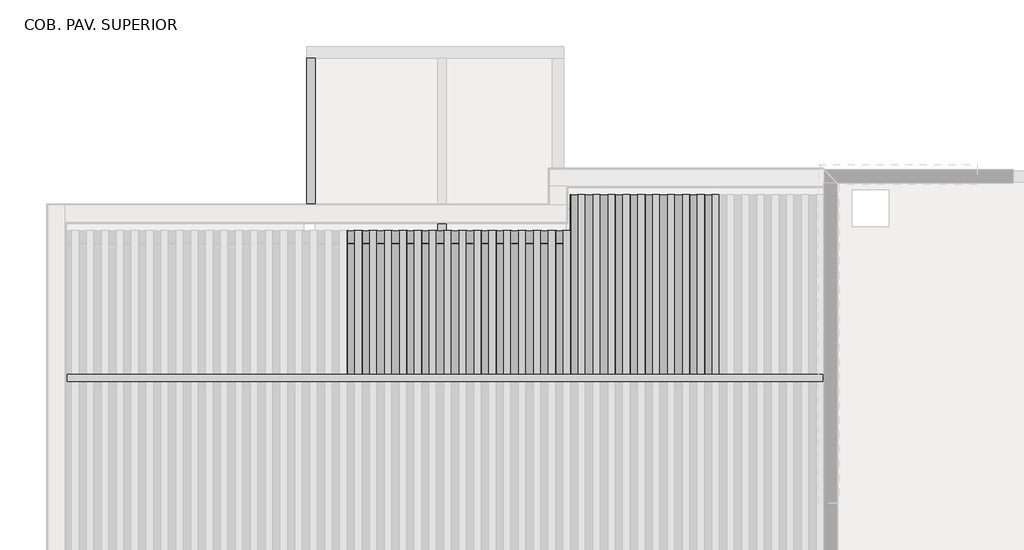
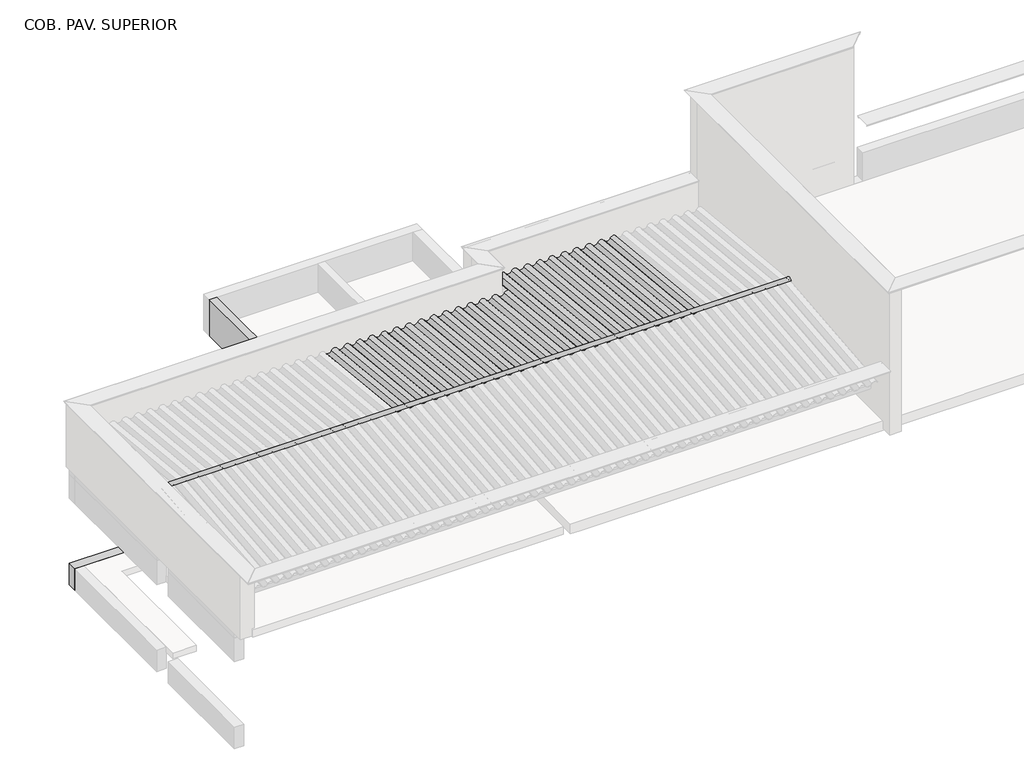
# One storey, part 4 of 7: 41 beams, 9 columns.
"""IFC4 building model written with IfcOpenShell, lengths in millimetres."""

import ifcopenshell
import ifcopenshell.guid

model = None  # the IFC model being written
_history = None  # IfcOwnerHistory: only IFC2X3 demands one
_inside = {}  # id of a spatial element -> (the spatial element, [elements in it])
_under = {}  # id of a project, library or spatial element -> (it, [spatial elements below it])
_declared = {}  # id of a project -> (the project, [libraries it declares])
_typed = {}  # id of a type object -> (the type object, [elements of that type])
_made_of = {}  # id of a material, layer set ... -> (it, [elements and type objects made of it])


def new_model(schema):
    """Start an empty IFC model of exactly this schema.

    Asked for "IFC4X3", IfcOpenShell would pick the latest addendum, in which some entities
    have other attributes; the version numbers below select the first issue.
    IFC2X3 requires an IfcOwnerHistory on every rooted entity: one is made here for all.
    """
    global model, _history
    if schema == "IFC4X3":
        model = ifcopenshell.file(schema_version=(4, 3, 0, 0))
    else:
        model = ifcopenshell.file(schema=schema)
    _inside.clear()
    _under.clear()
    _declared.clear()
    _typed.clear()
    _made_of.clear()
    _history = None
    if model.schema == "IFC2X3":
        org = make("IfcOrganization", Name="unknown")
        user = make(
            "IfcPersonAndOrganization",
            ThePerson=make("IfcPerson", FamilyName="unknown"),
            TheOrganization=org,
        )
        app = make(
            "IfcApplication",
            ApplicationDeveloper=org,
            Version="unknown",
            ApplicationFullName="unknown",
            ApplicationIdentifier="unknown",
        )
        _history = make(
            "IfcOwnerHistory",
            OwningUser=user,
            OwningApplication=app,
            ChangeAction="ADDED",
            CreationDate=0,
        )
    return model


def make(cls, **values):
    """One entity of the class cls with the attributes given. An attribute that is None is left unset."""
    return model.create_entity(
        cls, **{name: value for name, value in values.items() if value is not None}
    )


def rooted(cls, **values):
    """An entity with a GlobalId (a new one), such as an element, a storey or a relation."""
    return make(cls, GlobalId=ifcopenshell.guid.new(), OwnerHistory=_history, **values)


def si_unit(unit_type, name, prefix=None):
    """IfcSIUnit, for example si_unit("LENGTHUNIT", "METRE", prefix="MILLI")."""
    return make("IfcSIUnit", UnitType=unit_type, Prefix=prefix, Name=name)


def assignment(units):
    """IfcUnitAssignment: the units of a project."""
    return None if units is None else make("IfcUnitAssignment", Units=units)


def point(xyz):
    """IfcCartesianPoint."""
    return None if xyz is None else make("IfcCartesianPoint", Coordinates=xyz)


def direction(xyz):
    """IfcDirection."""
    return None if xyz is None else make("IfcDirection", DirectionRatios=xyz)


def frame(location, z_axis=None, x_axis=None):
    """IfcAxis2Placement3D, a coordinate frame: its origin and axes. An axis left out is left unset."""
    return make(
        "IfcAxis2Placement3D",
        Location=point(location),
        Axis=direction(z_axis),
        RefDirection=direction(x_axis),
    )


def frame_2d(location, x_axis=None):
    """IfcAxis2Placement2D, a coordinate frame in the plane: its origin and x axis."""
    return make(
        "IfcAxis2Placement2D", Location=point(location), RefDirection=direction(x_axis)
    )


def origin():
    """The frame at (0, 0, 0) with its axes left unset."""
    return frame((0.0, 0.0, 0.0))


def place(relative_to, where):
    """IfcLocalPlacement: puts the frame where relative to a parent placement (None: the world)."""
    return make(
        "IfcLocalPlacement", PlacementRelTo=relative_to, RelativePlacement=where
    )


def context(
    kind, dimensions, precision=None, world=None, true_north=None, identifier=None
):
    """IfcGeometricRepresentationContext, for example the 3D "Model" context."""
    return make(
        "IfcGeometricRepresentationContext",
        ContextIdentifier=identifier,
        ContextType=kind,
        CoordinateSpaceDimension=dimensions,
        Precision=precision,
        WorldCoordinateSystem=world,
        TrueNorth=true_north,
    )


def project(units=None, contexts=None):
    """IfcProject with its units and contexts."""
    return rooted(
        "IfcProject",
        Name="project",
        RepresentationContexts=contexts,
        UnitsInContext=assignment(units),
    )


def spatial(cls, under=None, at=None, **own):
    """A site, building, storey or space (cls), placed at a placement, below another one or the project."""
    s = rooted(cls, ObjectPlacement=at, **own)
    if under is not None:
        _under.setdefault(under.id(), (under, []))[1].append(s)
    return s


def polyline(points):
    """IfcPolyline through the points."""
    return make("IfcPolyline", Points=[point(p) for p in points])


def circle_curve(where, radius):
    """IfcCircle in the frame where."""
    return make("IfcCircle", Position=where, Radius=radius)


def trimmed(basis, trim1, trim2, sense, master):
    """IfcTrimmedCurve: the piece of a basis curve between two trims."""
    return make(
        "IfcTrimmedCurve",
        BasisCurve=basis,
        Trim1=trim1,
        Trim2=trim2,
        SenseAgreement=sense,
        MasterRepresentation=master,
    )


def segment(curve, same_sense, transition):
    """IfcCompositeCurveSegment."""
    return make(
        "IfcCompositeCurveSegment",
        Transition=transition,
        SameSense=same_sense,
        ParentCurve=curve,
    )


def composite_curve(segments, self_intersect=None):
    """IfcCompositeCurve: segments joined end to end."""
    return make("IfcCompositeCurve", Segments=segments, SelfIntersect=self_intersect)


def outline(outer, holes=None, kind="AREA"):
    """IfcArbitraryClosedProfileDef: a profile drawn as a closed curve; with holes, ...WithVoids."""
    if holes is None:
        return make("IfcArbitraryClosedProfileDef", ProfileType=kind, OuterCurve=outer)
    return make(
        "IfcArbitraryProfileDefWithVoids",
        ProfileType=kind,
        OuterCurve=outer,
        InnerCurves=holes,
    )


def extrude(swept, where, along, depth):
    """IfcExtrudedAreaSolid: the profile swept, set in the frame where, extruded along a direction by depth."""
    return make(
        "IfcExtrudedAreaSolid",
        SweptArea=swept,
        Position=where,
        ExtrudedDirection=direction(along),
        Depth=depth,
    )


def faces_of(points, faces, orient=None, outer=None):
    """IfcFace entities. A face is a list of loops; a loop is a list of indices into points, from 0.

    orient and outer hold one flag for each loop. By default every Orientation is true, the
    first loop of a face is its IfcFaceOuterBound and the others are IfcFaceBound.
    """
    made = []
    for i, loops in enumerate(faces):
        bounds = []
        for j, loop in enumerate(loops):
            is_outer = j == 0 if outer is None else outer[i][j]
            bounds.append(
                make(
                    "IfcFaceOuterBound" if is_outer else "IfcFaceBound",
                    Bound=make("IfcPolyLoop", Polygon=[points[k] for k in loop]),
                    Orientation=True if orient is None else orient[i][j],
                )
            )
        made.append(make("IfcFace", Bounds=bounds))
    return made


def faceted_brep(points, faces, orient=None, outer=None, voids=None):
    """IfcFacetedBrep: a solid bounded by flat faces; with voids (closed shells), ...WithVoids."""
    shared = [point(p) for p in points]
    hull = make("IfcClosedShell", CfsFaces=faces_of(shared, faces, orient, outer))
    if voids is None:
        return make("IfcFacetedBrep", Outer=hull)
    return make(
        "IfcFacetedBrepWithVoids",
        Outer=hull,
        Voids=[
            make(cls, CfsFaces=faces_of(shared, fs, o, b)) for cls, fs, o, b in voids
        ],
    )


def shape(context_of_items, identifier, shape_type, items):
    """IfcShapeRepresentation: the items that make up one representation, for example the "Body"."""
    return make(
        "IfcShapeRepresentation",
        ContextOfItems=context_of_items,
        RepresentationIdentifier=identifier,
        RepresentationType=shape_type,
        Items=items,
    )


def source(mapping_origin, context_of_items, identifier, shape_type, items):
    """IfcRepresentationMap: a shape defined once, which mapped items show again and again."""
    return make(
        "IfcRepresentationMap",
        MappingOrigin=mapping_origin,
        MappedRepresentation=shape(context_of_items, identifier, shape_type, items),
    )


def transform(
    local_origin,
    x_axis=None,
    y_axis=None,
    z_axis=None,
    scale=None,
    scale2=None,
    scale3=None,
    uniform=True,
):
    """IfcCartesianTransformationOperator3D, or its non-uniform kind. x_axis, y_axis, z_axis: its Axis1, 2, 3."""
    if uniform:
        return make(
            "IfcCartesianTransformationOperator3D",
            Axis1=direction(x_axis),
            Axis2=direction(y_axis),
            LocalOrigin=point(local_origin),
            Scale=scale,
            Axis3=direction(z_axis),
        )
    return make(
        "IfcCartesianTransformationOperator3DnonUniform",
        Axis1=direction(x_axis),
        Axis2=direction(y_axis),
        LocalOrigin=point(local_origin),
        Scale=scale,
        Axis3=direction(z_axis),
        Scale2=scale2,
        Scale3=scale3,
    )


def mapped(mapping_source, mapping_target):
    """IfcMappedItem: shows the shape of a source again, moved by a transform."""
    return make(
        "IfcMappedItem", MappingSource=mapping_source, MappingTarget=mapping_target
    )


def made_of(thing, what):
    """Note that an element or type object is made of a material, layer set ...; save() writes the relation."""
    if what is not None:
        _made_of.setdefault(what.id(), (what, []))[1].append(thing)
    return thing


def element(
    cls,
    number,
    at=None,
    inside=None,
    cuts=None,
    type_object=None,
    material=None,
    context=None,
    identifier="Body",
    shape_type=None,
    held_by="IfcProductDefinitionShape",
    body=None,
    shapes=None,
    **own,
):
    """One element of the class cls, such as IfcWall. Its Tag is "e" and its number.

    at: its placement. inside: the storey or other place that contains it. cuts: it is an
    opening in that element (IfcRelVoidsElement). A single representation is given by context,
    identifier, shape_type and body (its items); several are given by shapes. held_by: the class
    of the entity that holds the representations. save() writes the other relations.
    """
    e = rooted(cls, Tag="e%d" % number, ObjectPlacement=at, **own)
    if body is not None:
        shapes = [shape(context, identifier, shape_type, body)]
    if shapes is not None:
        e.Representation = make(held_by, Representations=shapes)
    if inside is not None:
        _inside.setdefault(inside.id(), (inside, []))[1].append(e)
    if cuts is not None:
        rooted(
            "IfcRelVoidsElement", RelatingBuildingElement=cuts, RelatedOpeningElement=e
        )
    if type_object is not None:
        _typed.setdefault(type_object.id(), (type_object, []))[1].append(e)
    return made_of(e, material)


def aggregate(whole, parts):
    """IfcRelAggregates: a whole, such as a stair, and the parts it consists of."""
    return rooted("IfcRelAggregates", RelatingObject=whole, RelatedObjects=parts)


def save(model, path):
    """Write the relations noted so far, then the file.

    IfcRelAggregates (storeys below a building ...), IfcRelContainedInSpatialStructure (elements
    in a storey), IfcRelDefinesByType, IfcRelAssociatesMaterial and IfcRelDeclares: one each for
    every whole, place, type object, material and project.
    """
    for whole, parts in _under.values():
        aggregate(whole, parts)
    for where, things in _inside.values():
        rooted(
            "IfcRelContainedInSpatialStructure",
            RelatedElements=things,
            RelatingStructure=where,
        )
    for kind, things in _typed.values():
        rooted("IfcRelDefinesByType", RelatedObjects=things, RelatingType=kind)
    for what, things in _made_of.values():
        rooted("IfcRelAssociatesMaterial", RelatedObjects=things, RelatingMaterial=what)
    for by, libraries in _declared.values():
        rooted("IfcRelDeclares", RelatingContext=by, RelatedDefinitions=libraries)
    model.write(path)


def cumeeira_telha_ondulada_fibrocimento_4a9e66c1(model_context):
    return source(origin(), model_context, "Body", "SweptSolid", [
        extrude(outline(composite_curve([segment(polyline([(58.3970135, 42.4437972), (53.9055884, 40.2467307)]), True, "CONTINUOUS"), segment(trimmed(circle_curve(frame_2d((-1.6029865, 13.0936483)), 61.7939461), [point((53.9055884, 40.2467307))], [point((-57.1115615, 40.2467307))], True, "CARTESIAN"), True, "CONTINUOUS"), segment(polyline([(-57.1115615, 40.2467307), (-61.6029865, 42.4437972)]), True, "CONTINUOUS"), segment(trimmed(circle_curve(frame_2d((-1.6029865, 13.0936483)), 66.7939461), [point((-61.6029865, 42.4437972))], [point((58.3970135, 42.4437972))], False, "CARTESIAN"), True, "CONTINUOUS")], self_intersect=False)), frame((-6200.0, 0.0, 0.0), z_axis=(1.0, 0.0, 0.0), x_axis=(0.0, 1.0, 0.0)), (0.0, 0.0, 1.0), 12400.0),
    ])


def viga_cumeeira_6x16cm_b61bb166(model_context):
    return source(origin(), model_context, "Body", "SweptSolid", [
        extrude(outline(polyline([(6210.0, 30.0), (6210.0, -30.0), (-6210.0, -30.0), (-6210.0, 30.0), (6210.0, 30.0)])), frame((0.0, 0.0, -80.0), z_axis=(0.0, 0.0, 1.0), x_axis=(1.0, 0.0, 0.0)), (0.0, 0.0, 1.0), 160.0),
    ])


def column_d505325c(model_context):
    return source(origin(), model_context, "Body", "SweptSolid", [
        extrude(outline(polyline([(30.0, 80.0), (30.0, -80.0), (-30.0, -80.0), (-30.0, 80.0), (30.0, 80.0)])), frame((0.0, 0.0, 6710.0), z_axis=(0.0, 0.0, 1.0), x_axis=(1.0, 0.0, 0.0)), (0.0, 0.0, 1.0), 750.0),
    ])


def column_df674f92(model_context):
    return source(origin(), model_context, "Body", "SweptSolid", [
        extrude(outline(polyline([(30.0, 80.0), (30.0, -80.0), (-30.0, -80.0), (-30.0, 80.0), (30.0, 80.0)])), frame((0.0, 0.0, 6710.0), z_axis=(0.0, 0.0, 1.0), x_axis=(1.0, 0.0, 0.0)), (0.0, 0.0, 1.0), 575.0),
    ])


def column_4db371bd(model_context):
    return source(origin(), model_context, "Body", "SweptSolid", [
        extrude(outline(polyline([(30.0, 80.0), (30.0, -80.0), (-30.0, -80.0), (-30.0, 80.0), (30.0, 80.0)])), frame((0.0, 0.0, 6710.0), z_axis=(0.0, 0.0, 1.0), x_axis=(1.0, 0.0, 0.0)), (0.0, 0.0, 1.0), 660.0),
    ])


model = new_model("IFC4")

# Units and contexts
model_context = context("Model", 3, world=origin())
ifc_project = project(units=[si_unit("LENGTHUNIT", "METRE", prefix="MILLI")], contexts=[model_context])

# Site, building, storey
site = spatial("IfcSite", under=ifc_project)
building = spatial("IfcBuilding", under=site)
storey = spatial("IfcBuildingStorey", under=building, Name="COB. PAV. SUPERIOR", Elevation=6650.0)

# Beams
placement = place(None, origin())
element("IfcBeam", 1, at=placement, inside=storey, context=model_context, shape_type="SweptSolid", body=[
    extrude(outline(polyline([(-6679.281307, -7711.5607799), (-6679.281307, -7831.5607799), (-8679.281307, -7831.5607799), (-8679.281307, -7711.5607799), (-6679.281307, -7711.5607799)])), frame((0.0, 0.0, 6650.0), z_axis=(0.0, 0.0, 1.0), x_axis=(1.0, 0.0, 0.0)), (0.0, 0.0, 1.0), 60.0),
])
element("IfcBeam", 2, at=placement, inside=storey, context=model_context, shape_type="SweptSolid", body=[
    extrude(outline(polyline([(-4679.281307, -7711.5607799), (-4679.281307, -7831.5607799), (-6679.281307, -7831.5607799), (-6679.281307, -7711.5607799), (-4679.281307, -7711.5607799)])), frame((0.0, 0.0, 6650.0), z_axis=(0.0, 0.0, 1.0), x_axis=(1.0, 0.0, 0.0)), (0.0, 0.0, 1.0), 60.0),
])
element("IfcBeam", 3, at=placement, inside=storey, context=model_context, shape_type="SweptSolid", body=[
    extrude(outline(polyline([(-2679.281307, -7711.5607799), (-2679.281307, -7831.5607799), (-4679.281307, -7831.5607799), (-4679.281307, -7711.5607799), (-2679.281307, -7711.5607799)])), frame((0.0, 0.0, 6650.0), z_axis=(0.0, 0.0, 1.0), x_axis=(1.0, 0.0, 0.0)), (0.0, 0.0, 1.0), 60.0),
])
element("IfcBeam", 4, at=placement, inside=storey, context=model_context, shape_type="SweptSolid", body=[
    extrude(outline(polyline([(-8779.281307, -5488.3211004), (-8779.281307, -5608.3211004), (-10679.281307, -5608.3211004), (-10679.281307, -5488.3211004), (-8779.281307, -5488.3211004)])), frame((0.0, 0.0, 6650.0), z_axis=(0.0, 0.0, 1.0), x_axis=(1.0, 0.0, 0.0)), (0.0, 0.0, 1.0), 60.0),
])
element("IfcBeam", 5, at=placement, inside=storey, context=model_context, shape_type="SweptSolid", body=[
    extrude(outline(polyline([(-6779.2813076, -5488.3211004), (-6779.2813076, -5608.3211004), (-8589.281307, -5608.3211004), (-8589.281307, -5488.3211004), (-6779.2813076, -5488.3211004)])), frame((0.0, 0.0, 6650.0), z_axis=(0.0, 0.0, 1.0), x_axis=(1.0, 0.0, 0.0)), (0.0, 0.0, 1.0), 60.0),
])
element("IfcBeam", 6, at=placement, inside=storey, context=model_context, shape_type="SweptSolid", body=[
    extrude(outline(polyline([(-4779.281307, -5488.3211004), (-4779.281307, -5608.3211004), (-6779.2813063, -5608.3211004), (-6779.2813063, -5488.3211004), (-4779.281307, -5488.3211004)])), frame((0.0, 0.0, 6650.0), z_axis=(0.0, 0.0, 1.0), x_axis=(1.0, 0.0, 0.0)), (0.0, 0.0, 1.0), 60.0),
])
element("IfcBeam", 7, at=placement, inside=storey, context=model_context, shape_type="SweptSolid", body=[
    extrude(outline(polyline([(-6840.281307, -6319.8711004), (-6840.281307, -6439.8711004), (-8589.281307, -6439.8711004), (-8589.281307, -6319.8711004), (-6840.281307, -6319.8711004)])), frame((0.0, 0.0, 6650.0), z_axis=(0.0, 0.0, 1.0), x_axis=(1.0, 0.0, 0.0)), (0.0, 0.0, 1.0), 60.0),
])
element("IfcBeam", 8, at=placement, inside=storey, context=model_context, shape_type="SweptSolid", body=[
    extrude(outline(polyline([(-4679.2813076, -6319.8711004), (-4679.2813076, -6439.8711004), (-6440.281307, -6439.8711004), (-6440.281307, -6319.8711004), (-4679.2813076, -6319.8711004)])), frame((0.0, 0.0, 6650.0), z_axis=(0.0, 0.0, 1.0), x_axis=(1.0, 0.0, 0.0)), (0.0, 0.0, 1.0), 60.0),
])
element("IfcBeam", 9, at=placement, inside=storey, context=model_context, shape_type="SweptSolid", body=[
    extrude(outline(polyline([(-2679.2813076, -6319.8711004), (-2679.2813076, -6439.8711004), (-4679.2813064, -6439.8711004), (-4679.2813064, -6319.8711004), (-2679.2813076, -6319.8711004)])), frame((0.0, 0.0, 6650.0), z_axis=(0.0, 0.0, 1.0), x_axis=(1.0, 0.0, 0.0)), (0.0, 0.0, 1.0), 60.0),
])
cumeeira_telha_ondulada_fibrocimento_shape = cumeeira_telha_ondulada_fibrocimento_4a9e66c1(model_context)
element("IfcBeam", 10, ObjectType="Cumeeira Telha Ondulada : Fibrocimento", at=placement, inside=storey, context=model_context, shape_type="MappedRepresentation", body=[
    mapped(cumeeira_telha_ondulada_fibrocimento_shape, transform((-6459.6793166, -7771.5607799, 7660.6251229), x_axis=(-1.0, 0.0, 0.0), y_axis=(0.0, -1.0, 0.0), z_axis=(0.0, 0.0, 1.0))),
])
element("IfcBeam", 11, ObjectType="TQS - Viga retangular : 14.0 x 76.0", at=placement, inside=storey, context=model_context, shape_type="Brep", body=[
    faceted_brep([(-8730.281307, -4975.5699847, 7050.0), (-8590.281307, -4975.5699847, 7050.0), (-8590.281307, -2515.5699847, 7050.0), (-8730.281307, -2515.5699847, 7050.0), (-8590.281307, -4975.5699847, 6450.0), (-8590.281307, -4975.5699847, 6290.0), (-8590.281307, -2515.5699847, 6290.0), (-8590.281307, -2515.5699847, 6450.0), (-8730.281307, -4975.5699847, 6290.0), (-8730.281307, -2515.5699847, 6290.0)], [[[0, 1, 2, 3]], [[1, 4, 5, 6, 7, 2]], [[5, 8, 9, 6]], [[8, 0, 3, 9]], [[1, 0, 8, 5, 4]], [[3, 2, 7, 6, 9]]]),
])
element("IfcBeam", 12, ObjectType="TQS - Viga retangular : 14.0 x 76.0", at=placement, inside=storey, context=model_context, shape_type="Brep", body=[
    faceted_brep([(-6440.281307, -5165.5699847, 7050.0), (-6580.281307, -5165.5699847, 7050.0), (-6580.281307, -6413.3699847, 7050.0), (-6440.281307, -6413.3699847, 7050.0), (-6440.281307, -5165.5699847, 6290.0), (-6440.281307, -5165.5699847, 6450.0), (-6440.281307, -5165.5699847, 6650.0), (-6440.281307, -6413.3699847, 6290.0), (-6580.281307, -5165.5699847, 6290.0), (-6580.281307, -6413.3699847, 6290.0), (-6580.281307, -5165.5699847, 6450.0), (-6580.281307, -6413.3699847, 6450.0)], [[[0, 1, 2, 3]], [[4, 5, 6, 0, 3, 7]], [[8, 4, 7, 9]], [[1, 10, 8, 9, 11, 2]], [[1, 0, 6, 5, 4, 8, 10]], [[2, 11, 9, 7, 3]]]),
])
element("IfcBeam", 13, ObjectType="TQS - Viga retangular : 19.0 x 45.0", at=placement, inside=storey, context=model_context, shape_type="Brep", body=[
    faceted_brep([(-8779.281307, -5165.5699847, 4480.0), (-8779.281307, -4975.5699847, 4480.0), (-12930.2813069, -4975.5699847, 4480.0), (-12930.2813069, -5165.5699847, 4480.0), (-12740.2813069, -5165.5699847, 4480.0), (-9711.481307, -5165.5699847, 4480.0), (-8779.281307, -5165.5699847, 4030.0), (-12930.2813069, -5165.5699847, 4030.0), (-12740.2813069, -5165.5699847, 4030.0), (-8779.281307, -4975.5699847, 4030.0), (-12930.2813069, -4975.5699847, 4030.0)], [[[0, 1, 2, 3, 4, 5]], [[6, 0, 5, 4, 3, 7, 8]], [[9, 6, 8, 7, 10]], [[1, 9, 10, 2]], [[1, 0, 6, 9]], [[3, 2, 10, 7]]]),
])
element("IfcBeam", 14, ObjectType="TQS - Viga retangular : 19.0 x 96.0", at=placement, inside=storey, context=model_context, shape_type="Brep", body=[
    faceted_brep([(-4702.281307, -5165.5699847, 7250.0), (-4512.281307, -5165.5699847, 7250.0), (-4512.281307, -4565.5699847, 7250.0), (-4512.281307, -4375.5699847, 7250.0), (-4702.281307, -4375.5699847, 7250.0), (-4702.281307, -4975.5699847, 7250.0), (-4512.281307, -4375.5699847, 6290.0), (-4512.281307, -4375.5699847, 6450.0), (-4512.281307, -4375.5699847, 7050.0), (-4512.281307, -5165.5699847, 6650.0), (-4512.281307, -5165.5699847, 6450.0), (-4512.281307, -5165.5699847, 6290.0), (-4702.281307, -5165.5699847, 6290.0), (-4702.281307, -4975.5699847, 6290.0), (-4702.281307, -4375.5699847, 6290.0), (-4702.281307, -4375.5699847, 7050.0), (-4702.281307, -5165.5699847, 6450.0), (-4702.281307, -5165.5699847, 6650.0)], [[[0, 1, 2, 3, 4, 5]], [[6, 7, 8, 3, 2, 1, 9, 10, 11]], [[11, 12, 13, 14, 6]], [[4, 15, 14, 13, 12, 16, 17, 0, 5]], [[1, 0, 17, 16, 12, 11, 10, 9]], [[4, 3, 8, 7, 6, 14, 15]]]),
])
element("IfcBeam", 15, ObjectType="TQS - Viga retangular : 19.0 x 96.0", at=placement, inside=storey, context=model_context, shape_type="Brep", body=[
    faceted_brep([(-6440.281307, -4975.5699847, 7250.0), (-6440.281307, -5165.5699847, 7250.0), (-4702.281307, -5165.5699847, 7250.0), (-4702.281307, -4975.5699847, 7250.0), (-6440.281307, -5165.5699847, 6650.0), (-6440.281307, -5165.5699847, 6450.0), (-6440.281307, -5165.5699847, 6290.0), (-4702.281307, -5165.5699847, 6290.0), (-4702.281307, -5165.5699847, 6450.0), (-4702.281307, -5165.5699847, 6650.0), (-6440.281307, -4975.5699847, 6290.0), (-4702.281307, -4975.5699847, 6290.0), (-6440.281307, -4975.5699847, 6450.0), (-4702.281307, -4975.5699847, 6450.0)], [[[0, 1, 2, 3]], [[2, 1, 4, 5, 6, 7, 8, 9]], [[6, 10, 11, 7]], [[10, 12, 0, 3, 13, 11]], [[1, 0, 12, 10, 6, 5, 4]], [[3, 2, 9, 8, 7, 11, 13]]]),
    faceted_brep([(-8589.281307, -5165.5699847, 7250.0), (-8589.281307, -4975.5699847, 7250.0), (-8589.281307, -4975.5699847, 6290.0), (-8589.281307, -5165.5699847, 6290.0), (-8589.281307, -5165.5699847, 6450.0), (-6630.281307, -4975.5699847, 7250.0), (-6630.281307, -5165.5699847, 7250.0), (-6630.281307, -5165.5699847, 6290.0), (-6630.281307, -4975.5699847, 6290.0)], [[[0, 1, 2, 3, 4]], [[5, 6, 7, 8]], [[1, 0, 6, 5]], [[0, 4, 3, 7, 6]], [[3, 2, 8, 7]], [[2, 1, 5, 8]]]),
])
element("IfcBeam", 16, ObjectType="Telha Ondulada : Fibrocimento", at=placement, inside=storey, context=model_context, shape_type="SweptSolid", body=[
    extrude(outline(composite_curve([segment(trimmed(circle_curve(frame_2d((-58.7002978, -53.2060539)), 66.7939461), [point((-29.3501489, 6.7939461))], [point((-29.3501489, -113.2060539))], False, "CARTESIAN"), True, "CONTINUOUS"), segment(polyline([(-29.3501489, -113.2060539), (-31.5472154, -108.7146289)]), True, "CONTINUOUS"), segment(trimmed(circle_curve(frame_2d((-58.7002978, -53.2060539)), 61.7939461), [point((-31.5472154, -108.7146289))], [point((-31.5472154, 2.3025211))], True, "CARTESIAN"), True, "CONTINUOUS"), segment(trimmed(circle_curve(frame_2d((0.0, 66.7939461)), 71.7939461), [point((-31.5472154, 2.3025211))], [point((-31.5472154, 131.2853711))], False, "CARTESIAN"), True, "CONTINUOUS"), segment(polyline([(-31.5472154, 131.2853711), (-29.3501489, 126.7939461)]), True, "CONTINUOUS"), segment(trimmed(circle_curve(frame_2d((0.0, 66.7939461)), 66.7939461), [point((-29.3501489, 126.7939461))], [point((-29.3501489, 6.7939461))], True, "CARTESIAN"), True, "CONTINUOUS")], self_intersect=False)), frame((-7939.8843743, -5348.1805671, 7453.4315886), z_axis=(0.0, -0.9950371902099893, 0.09950371902099772), x_axis=(0.0, 0.09950371902099772, 0.9950371902099893)), (0.0, 0.0, 1.0), 2425.2918406),
])
element("IfcBeam", 17, ObjectType="Telha Ondulada : Fibrocimento", at=placement, inside=storey, context=model_context, shape_type="SweptSolid", body=[
    extrude(outline(composite_curve([segment(trimmed(circle_curve(frame_2d((-58.7002978, -53.2060539)), 66.7939461), [point((-29.3501489, 6.7939461))], [point((-29.3501489, -113.2060539))], False, "CARTESIAN"), True, "CONTINUOUS"), segment(polyline([(-29.3501489, -113.2060539), (-31.5472154, -108.7146289)]), True, "CONTINUOUS"), segment(trimmed(circle_curve(frame_2d((-58.7002978, -53.2060539)), 61.7939461), [point((-31.5472154, -108.7146289))], [point((-31.5472154, 2.3025211))], True, "CARTESIAN"), True, "CONTINUOUS"), segment(trimmed(circle_curve(frame_2d((0.0, 66.7939461)), 71.7939461), [point((-31.5472154, 2.3025211))], [point((-31.5472154, 131.2853711))], False, "CARTESIAN"), True, "CONTINUOUS"), segment(polyline([(-31.5472154, 131.2853711), (-29.3501489, 126.7939461)]), True, "CONTINUOUS"), segment(trimmed(circle_curve(frame_2d((0.0, 66.7939461)), 66.7939461), [point((-29.3501489, 126.7939461))], [point((-29.3501489, 6.7939461))], True, "CARTESIAN"), True, "CONTINUOUS")], self_intersect=False)), frame((-7695.3843743, -5348.1805671, 7453.4315886), z_axis=(0.0, -0.9950371902099893, 0.09950371902099772), x_axis=(0.0, 0.09950371902099772, 0.9950371902099893)), (0.0, 0.0, 1.0), 2425.2918406),
])
element("IfcBeam", 18, ObjectType="Telha Ondulada : Fibrocimento", at=placement, inside=storey, context=model_context, shape_type="SweptSolid", body=[
    extrude(outline(composite_curve([segment(trimmed(circle_curve(frame_2d((-58.7002978, -53.2060539)), 66.7939461), [point((-29.3501489, 6.7939461))], [point((-29.3501489, -113.2060539))], False, "CARTESIAN"), True, "CONTINUOUS"), segment(polyline([(-29.3501489, -113.2060539), (-31.5472154, -108.7146289)]), True, "CONTINUOUS"), segment(trimmed(circle_curve(frame_2d((-58.7002978, -53.2060539)), 61.7939461), [point((-31.5472154, -108.7146289))], [point((-31.5472154, 2.3025211))], True, "CARTESIAN"), True, "CONTINUOUS"), segment(trimmed(circle_curve(frame_2d((0.0, 66.7939461)), 71.7939461), [point((-31.5472154, 2.3025211))], [point((-31.5472154, 131.2853711))], False, "CARTESIAN"), True, "CONTINUOUS"), segment(polyline([(-31.5472154, 131.2853711), (-29.3501489, 126.7939461)]), True, "CONTINUOUS"), segment(trimmed(circle_curve(frame_2d((0.0, 66.7939461)), 66.7939461), [point((-29.3501489, 126.7939461))], [point((-29.3501489, 6.7939461))], True, "CARTESIAN"), True, "CONTINUOUS")], self_intersect=False)), frame((-7450.8843743, -5348.1805671, 7453.4315886), z_axis=(0.0, -0.9950371902099893, 0.09950371902099768), x_axis=(0.0, 0.09950371902099768, 0.9950371902099893)), (0.0, 0.0, 1.0), 2425.2918406),
])
element("IfcBeam", 19, ObjectType="Telha Ondulada : Fibrocimento", at=placement, inside=storey, context=model_context, shape_type="SweptSolid", body=[
    extrude(outline(composite_curve([segment(trimmed(circle_curve(frame_2d((-58.7002978, -53.2060539)), 66.7939461), [point((-29.3501489, 6.7939461))], [point((-29.3501489, -113.2060539))], False, "CARTESIAN"), True, "CONTINUOUS"), segment(polyline([(-29.3501489, -113.2060539), (-31.5472154, -108.7146289)]), True, "CONTINUOUS"), segment(trimmed(circle_curve(frame_2d((-58.7002978, -53.2060539)), 61.7939461), [point((-31.5472154, -108.7146289))], [point((-31.5472154, 2.3025211))], True, "CARTESIAN"), True, "CONTINUOUS"), segment(trimmed(circle_curve(frame_2d((0.0, 66.7939461)), 71.7939461), [point((-31.5472154, 2.3025211))], [point((-31.5472154, 131.2853711))], False, "CARTESIAN"), True, "CONTINUOUS"), segment(polyline([(-31.5472154, 131.2853711), (-29.3501489, 126.7939461)]), True, "CONTINUOUS"), segment(trimmed(circle_curve(frame_2d((0.0, 66.7939461)), 66.7939461), [point((-29.3501489, 126.7939461))], [point((-29.3501489, 6.7939461))], True, "CARTESIAN"), True, "CONTINUOUS")], self_intersect=False)), frame((-7206.3843743, -5348.1805671, 7453.4315886), z_axis=(0.0, -0.9950371902099893, 0.09950371902099768), x_axis=(0.0, 0.09950371902099768, 0.9950371902099893)), (0.0, 0.0, 1.0), 2425.2918406),
])
element("IfcBeam", 20, ObjectType="Telha Ondulada : Fibrocimento", at=placement, inside=storey, context=model_context, shape_type="SweptSolid", body=[
    extrude(outline(composite_curve([segment(trimmed(circle_curve(frame_2d((-58.7002978, -53.2060539)), 66.7939461), [point((-29.3501489, 6.7939461))], [point((-29.3501489, -113.2060539))], False, "CARTESIAN"), True, "CONTINUOUS"), segment(polyline([(-29.3501489, -113.2060539), (-31.5472154, -108.7146289)]), True, "CONTINUOUS"), segment(trimmed(circle_curve(frame_2d((-58.7002978, -53.2060539)), 61.7939461), [point((-31.5472154, -108.7146289))], [point((-31.5472154, 2.3025211))], True, "CARTESIAN"), True, "CONTINUOUS"), segment(trimmed(circle_curve(frame_2d((0.0, 66.7939461)), 71.7939461), [point((-31.5472154, 2.3025211))], [point((-31.5472154, 131.2853711))], False, "CARTESIAN"), True, "CONTINUOUS"), segment(polyline([(-31.5472154, 131.2853711), (-29.3501489, 126.7939461)]), True, "CONTINUOUS"), segment(trimmed(circle_curve(frame_2d((0.0, 66.7939461)), 66.7939461), [point((-29.3501489, 126.7939461))], [point((-29.3501489, 6.7939461))], True, "CARTESIAN"), True, "CONTINUOUS")], self_intersect=False)), frame((-6961.8843743, -5348.1805671, 7453.4315886), z_axis=(0.0, -0.9950371902099893, 0.09950371902099768), x_axis=(0.0, 0.09950371902099768, 0.9950371902099893)), (0.0, 0.0, 1.0), 2425.2918406),
])
element("IfcBeam", 21, ObjectType="Telha Ondulada : Fibrocimento", at=placement, inside=storey, context=model_context, shape_type="SweptSolid", body=[
    extrude(outline(composite_curve([segment(trimmed(circle_curve(frame_2d((-58.7002978, -53.2060539)), 66.7939461), [point((-29.3501489, 6.7939461))], [point((-29.3501489, -113.2060539))], False, "CARTESIAN"), True, "CONTINUOUS"), segment(polyline([(-29.3501489, -113.2060539), (-31.5472154, -108.7146289)]), True, "CONTINUOUS"), segment(trimmed(circle_curve(frame_2d((-58.7002978, -53.2060539)), 61.7939461), [point((-31.5472154, -108.7146289))], [point((-31.5472154, 2.3025211))], True, "CARTESIAN"), True, "CONTINUOUS"), segment(trimmed(circle_curve(frame_2d((0.0, 66.7939461)), 71.7939461), [point((-31.5472154, 2.3025211))], [point((-31.5472154, 131.2853711))], False, "CARTESIAN"), True, "CONTINUOUS"), segment(polyline([(-31.5472154, 131.2853711), (-29.3501489, 126.7939461)]), True, "CONTINUOUS"), segment(trimmed(circle_curve(frame_2d((0.0, 66.7939461)), 66.7939461), [point((-29.3501489, 126.7939461))], [point((-29.3501489, 6.7939461))], True, "CARTESIAN"), True, "CONTINUOUS")], self_intersect=False)), frame((-6717.3843743, -5348.1805671, 7453.4315886), z_axis=(0.0, -0.9950371902099893, 0.09950371902099768), x_axis=(0.0, 0.09950371902099768, 0.9950371902099893)), (0.0, 0.0, 1.0), 2425.2918406),
])
element("IfcBeam", 22, ObjectType="Telha Ondulada : Fibrocimento", at=placement, inside=storey, context=model_context, shape_type="SweptSolid", body=[
    extrude(outline(composite_curve([segment(trimmed(circle_curve(frame_2d((-58.7002978, -53.2060539)), 66.7939461), [point((-29.3501489, 6.7939461))], [point((-29.3501489, -113.2060539))], False, "CARTESIAN"), True, "CONTINUOUS"), segment(polyline([(-29.3501489, -113.2060539), (-31.5472154, -108.7146289)]), True, "CONTINUOUS"), segment(trimmed(circle_curve(frame_2d((-58.7002978, -53.2060539)), 61.7939461), [point((-31.5472154, -108.7146289))], [point((-31.5472154, 2.3025211))], True, "CARTESIAN"), True, "CONTINUOUS"), segment(trimmed(circle_curve(frame_2d((0.0, 66.7939461)), 71.7939461), [point((-31.5472154, 2.3025211))], [point((-31.5472154, 131.2853711))], False, "CARTESIAN"), True, "CONTINUOUS"), segment(polyline([(-31.5472154, 131.2853711), (-29.3501489, 126.7939461)]), True, "CONTINUOUS"), segment(trimmed(circle_curve(frame_2d((0.0, 66.7939461)), 66.7939461), [point((-29.3501489, 126.7939461))], [point((-29.3501489, 6.7939461))], True, "CARTESIAN"), True, "CONTINUOUS")], self_intersect=False)), frame((-6472.8843743, -5348.1805671, 7453.4315886), z_axis=(0.0, -0.9950371902099893, 0.09950371902099772), x_axis=(0.0, 0.09950371902099772, 0.9950371902099893)), (0.0, 0.0, 1.0), 2425.2918406),
])
element("IfcBeam", 23, ObjectType="Telha Ondulada : Fibrocimento", at=placement, inside=storey, context=model_context, shape_type="SweptSolid", body=[
    extrude(outline(composite_curve([segment(trimmed(circle_curve(frame_2d((-58.7002978, -53.2060539)), 66.7939461), [point((-29.3501489, 6.7939461))], [point((-29.3501489, -113.2060539))], False, "CARTESIAN"), True, "CONTINUOUS"), segment(polyline([(-29.3501489, -113.2060539), (-31.5472154, -108.7146289)]), True, "CONTINUOUS"), segment(trimmed(circle_curve(frame_2d((-58.7002978, -53.2060539)), 61.7939461), [point((-31.5472154, -108.7146289))], [point((-31.5472154, 2.3025211))], True, "CARTESIAN"), True, "CONTINUOUS"), segment(trimmed(circle_curve(frame_2d((0.0, 66.7939461)), 71.7939461), [point((-31.5472154, 2.3025211))], [point((-31.5472154, 131.2853711))], False, "CARTESIAN"), True, "CONTINUOUS"), segment(polyline([(-31.5472154, 131.2853711), (-29.3501489, 126.7939461)]), True, "CONTINUOUS"), segment(trimmed(circle_curve(frame_2d((0.0, 66.7939461)), 66.7939461), [point((-29.3501489, 126.7939461))], [point((-29.3501489, 6.7939461))], True, "CARTESIAN"), True, "CONTINUOUS")], self_intersect=False)), frame((-6228.3843743, -5348.1805671, 7453.4315886), z_axis=(0.0, -0.9950371902099893, 0.09950371902099768), x_axis=(0.0, 0.09950371902099768, 0.9950371902099893)), (0.0, 0.0, 1.0), 2425.2918406),
])
element("IfcBeam", 24, ObjectType="Telha Ondulada : Fibrocimento", at=placement, inside=storey, context=model_context, shape_type="SweptSolid", body=[
    extrude(outline(composite_curve([segment(trimmed(circle_curve(frame_2d((-58.7002978, -53.2060539)), 66.7939461), [point((-29.3501489, 6.7939461))], [point((-29.3501489, -113.2060539))], False, "CARTESIAN"), True, "CONTINUOUS"), segment(polyline([(-29.3501489, -113.2060539), (-31.5472154, -108.7146289)]), True, "CONTINUOUS"), segment(trimmed(circle_curve(frame_2d((-58.7002978, -53.2060539)), 61.7939461), [point((-31.5472154, -108.7146289))], [point((-31.5472154, 2.3025211))], True, "CARTESIAN"), True, "CONTINUOUS"), segment(trimmed(circle_curve(frame_2d((0.0, 66.7939461)), 71.7939461), [point((-31.5472154, 2.3025211))], [point((-31.5472154, 131.2853711))], False, "CARTESIAN"), True, "CONTINUOUS"), segment(polyline([(-31.5472154, 131.2853711), (-29.3501489, 126.7939461)]), True, "CONTINUOUS"), segment(trimmed(circle_curve(frame_2d((0.0, 66.7939461)), 66.7939461), [point((-29.3501489, 126.7939461))], [point((-29.3501489, 6.7939461))], True, "CARTESIAN"), True, "CONTINUOUS")], self_intersect=False)), frame((-5983.8843743, -5348.1805671, 7453.4315886), z_axis=(0.0, -0.9950371902099893, 0.09950371902099772), x_axis=(0.0, 0.09950371902099772, 0.9950371902099893)), (0.0, 0.0, 1.0), 2425.2918406),
])
element("IfcBeam", 25, ObjectType="Telha Ondulada : Fibrocimento", at=placement, inside=storey, context=model_context, shape_type="SweptSolid", body=[
    extrude(outline(composite_curve([segment(trimmed(circle_curve(frame_2d((-58.7002978, -53.2060539)), 66.7939461), [point((-29.3501489, 6.7939461))], [point((-29.3501489, -113.2060539))], False, "CARTESIAN"), True, "CONTINUOUS"), segment(polyline([(-29.3501489, -113.2060539), (-31.5472154, -108.7146289)]), True, "CONTINUOUS"), segment(trimmed(circle_curve(frame_2d((-58.7002978, -53.2060539)), 61.7939461), [point((-31.5472154, -108.7146289))], [point((-31.5472154, 2.3025211))], True, "CARTESIAN"), True, "CONTINUOUS"), segment(trimmed(circle_curve(frame_2d((0.0, 66.7939461)), 71.7939461), [point((-31.5472154, 2.3025211))], [point((-31.5472154, 131.2853711))], False, "CARTESIAN"), True, "CONTINUOUS"), segment(polyline([(-31.5472154, 131.2853711), (-29.3501489, 126.7939461)]), True, "CONTINUOUS"), segment(trimmed(circle_curve(frame_2d((0.0, 66.7939461)), 66.7939461), [point((-29.3501489, 126.7939461))], [point((-29.3501489, 6.7939461))], True, "CARTESIAN"), True, "CONTINUOUS")], self_intersect=False)), frame((-5739.3843743, -5348.1805671, 7453.4315886), z_axis=(0.0, -0.9950371902099893, 0.09950371902099772), x_axis=(0.0, 0.09950371902099772, 0.9950371902099893)), (0.0, 0.0, 1.0), 2425.2918406),
])
element("IfcBeam", 26, ObjectType="Telha Ondulada : Fibrocimento", at=placement, inside=storey, context=model_context, shape_type="SweptSolid", body=[
    extrude(outline(composite_curve([segment(trimmed(circle_curve(frame_2d((-58.7002978, -53.2060539)), 66.7939461), [point((-29.3501489, 6.7939461))], [point((-29.3501489, -113.2060539))], False, "CARTESIAN"), True, "CONTINUOUS"), segment(polyline([(-29.3501489, -113.2060539), (-31.5472154, -108.7146289)]), True, "CONTINUOUS"), segment(trimmed(circle_curve(frame_2d((-58.7002978, -53.2060539)), 61.7939461), [point((-31.5472154, -108.7146289))], [point((-31.5472154, 2.3025211))], True, "CARTESIAN"), True, "CONTINUOUS"), segment(trimmed(circle_curve(frame_2d((0.0, 66.7939461)), 71.7939461), [point((-31.5472154, 2.3025211))], [point((-31.5472154, 131.2853711))], False, "CARTESIAN"), True, "CONTINUOUS"), segment(polyline([(-31.5472154, 131.2853711), (-29.3501489, 126.7939461)]), True, "CONTINUOUS"), segment(trimmed(circle_curve(frame_2d((0.0, 66.7939461)), 66.7939461), [point((-29.3501489, 126.7939461))], [point((-29.3501489, 6.7939461))], True, "CARTESIAN"), True, "CONTINUOUS")], self_intersect=False)), frame((-5494.8843743, -5348.1805671, 7453.4315886), z_axis=(0.0, -0.9950371902099893, 0.09950371902099768), x_axis=(0.0, 0.09950371902099768, 0.9950371902099893)), (0.0, 0.0, 1.0), 2425.2918406),
])
element("IfcBeam", 27, ObjectType="Telha Ondulada : Fibrocimento", at=placement, inside=storey, context=model_context, shape_type="SweptSolid", body=[
    extrude(outline(composite_curve([segment(trimmed(circle_curve(frame_2d((-58.7002978, -53.2060539)), 66.7939461), [point((-29.3501489, 6.7939461))], [point((-29.3501489, -113.2060539))], False, "CARTESIAN"), True, "CONTINUOUS"), segment(polyline([(-29.3501489, -113.2060539), (-31.5472154, -108.7146289)]), True, "CONTINUOUS"), segment(trimmed(circle_curve(frame_2d((-58.7002978, -53.2060539)), 61.7939461), [point((-31.5472154, -108.7146289))], [point((-31.5472154, 2.3025211))], True, "CARTESIAN"), True, "CONTINUOUS"), segment(trimmed(circle_curve(frame_2d((0.0, 66.7939461)), 71.7939461), [point((-31.5472154, 2.3025211))], [point((-31.5472154, 131.2853711))], False, "CARTESIAN"), True, "CONTINUOUS"), segment(polyline([(-31.5472154, 131.2853711), (-29.3501489, 126.7939461)]), True, "CONTINUOUS"), segment(trimmed(circle_curve(frame_2d((0.0, 66.7939461)), 66.7939461), [point((-29.3501489, 126.7939461))], [point((-29.3501489, 6.7939461))], True, "CARTESIAN"), True, "CONTINUOUS")], self_intersect=False)), frame((-5250.3843743, -5348.1805671, 7453.4315886), z_axis=(0.0, -0.9950371902099893, 0.09950371902099772), x_axis=(0.0, 0.09950371902099772, 0.9950371902099893)), (0.0, 0.0, 1.0), 2425.2918406),
])
element("IfcBeam", 28, ObjectType="Telha Ondulada : Fibrocimento", at=placement, inside=storey, context=model_context, shape_type="SweptSolid", body=[
    extrude(outline(composite_curve([segment(trimmed(circle_curve(frame_2d((-58.7002978, -53.2060539)), 66.7939461), [point((-29.3501489, 6.7939461))], [point((-29.3501489, -113.2060539))], False, "CARTESIAN"), True, "CONTINUOUS"), segment(polyline([(-29.3501489, -113.2060539), (-31.5472154, -108.7146289)]), True, "CONTINUOUS"), segment(trimmed(circle_curve(frame_2d((-58.7002978, -53.2060539)), 61.7939461), [point((-31.5472154, -108.7146289))], [point((-31.5472154, 2.3025211))], True, "CARTESIAN"), True, "CONTINUOUS"), segment(trimmed(circle_curve(frame_2d((0.0, 66.7939461)), 71.7939461), [point((-31.5472154, 2.3025211))], [point((-31.5472154, 131.2853711))], False, "CARTESIAN"), True, "CONTINUOUS"), segment(polyline([(-31.5472154, 131.2853711), (-29.3501489, 126.7939461)]), True, "CONTINUOUS"), segment(trimmed(circle_curve(frame_2d((0.0, 66.7939461)), 66.7939461), [point((-29.3501489, 126.7939461))], [point((-29.3501489, 6.7939461))], True, "CARTESIAN"), True, "CONTINUOUS")], self_intersect=False)), frame((-5005.8843743, -5348.1805671, 7453.4315886), z_axis=(0.0, -0.9950371902099893, 0.09950371902099772), x_axis=(0.0, 0.09950371902099772, 0.9950371902099893)), (0.0, 0.0, 1.0), 2425.2918406),
])
element("IfcBeam", 29, ObjectType="Telha Ondulada : Fibrocimento", at=placement, inside=storey, context=model_context, shape_type="SweptSolid", body=[
    extrude(outline(composite_curve([segment(trimmed(circle_curve(frame_2d((-58.7002978, -53.2060539)), 66.7939461), [point((-29.3501489, 6.7939461))], [point((-29.3501489, -113.2060539))], False, "CARTESIAN"), True, "CONTINUOUS"), segment(polyline([(-29.3501489, -113.2060539), (-31.5472154, -108.7146289)]), True, "CONTINUOUS"), segment(trimmed(circle_curve(frame_2d((-58.7002978, -53.2060539)), 61.7939461), [point((-31.5472154, -108.7146289))], [point((-31.5472154, 2.3025211))], True, "CARTESIAN"), True, "CONTINUOUS"), segment(trimmed(circle_curve(frame_2d((0.0, 66.7939461)), 71.7939461), [point((-31.5472154, 2.3025211))], [point((-31.5472154, 131.2853711))], False, "CARTESIAN"), True, "CONTINUOUS"), segment(polyline([(-31.5472154, 131.2853711), (-29.3501489, 126.7939461)]), True, "CONTINUOUS"), segment(trimmed(circle_curve(frame_2d((0.0, 66.7939461)), 66.7939461), [point((-29.3501489, 126.7939461))], [point((-29.3501489, 6.7939461))], True, "CARTESIAN"), True, "CONTINUOUS")], self_intersect=False)), frame((-4761.3843743, -5348.1805671, 7453.4315886), z_axis=(0.0, -0.9950371902099893, 0.09950371902099768), x_axis=(0.0, 0.09950371902099768, 0.9950371902099893)), (0.0, 0.0, 1.0), 2425.2918406),
])
element("IfcBeam", 30, ObjectType="Telha Ondulada : Fibrocimento", at=placement, inside=storey, context=model_context, shape_type="SweptSolid", body=[
    extrude(outline(composite_curve([segment(trimmed(circle_curve(frame_2d((-58.7002978, -53.2060539)), 66.7939461), [point((-29.3501489, 6.7939461))], [point((-29.3501489, -113.2060539))], False, "CARTESIAN"), True, "CONTINUOUS"), segment(polyline([(-29.3501489, -113.2060539), (-31.5472154, -108.7146289)]), True, "CONTINUOUS"), segment(trimmed(circle_curve(frame_2d((-58.7002978, -53.2060539)), 61.7939461), [point((-31.5472154, -108.7146289))], [point((-31.5472154, 2.3025211))], True, "CARTESIAN"), True, "CONTINUOUS"), segment(trimmed(circle_curve(frame_2d((0.0, 66.7939461)), 71.7939461), [point((-31.5472154, 2.3025211))], [point((-31.5472154, 131.2853711))], False, "CARTESIAN"), True, "CONTINUOUS"), segment(polyline([(-31.5472154, 131.2853711), (-29.3501489, 126.7939461)]), True, "CONTINUOUS"), segment(trimmed(circle_curve(frame_2d((0.0, 66.7939461)), 66.7939461), [point((-29.3501489, 126.7939461))], [point((-29.3501489, 6.7939461))], True, "CARTESIAN"), True, "CONTINUOUS")], self_intersect=False)), frame((-4516.8843743, -5348.1805671, 7453.4315886), z_axis=(0.0, -0.9950371902099893, 0.09950371902099772), x_axis=(0.0, 0.09950371902099772, 0.9950371902099893)), (0.0, 0.0, 1.0), 2425.2918406),
])
element("IfcBeam", 31, ObjectType="Telha Ondulada : Fibrocimento", at=placement, inside=storey, context=model_context, shape_type="SweptSolid", body=[
    extrude(outline(composite_curve([segment(trimmed(circle_curve(frame_2d((-58.7002978, -53.2060539)), 66.7939461), [point((-29.3501489, 6.7939461))], [point((-29.3501489, -113.2060539))], False, "CARTESIAN"), True, "CONTINUOUS"), segment(polyline([(-29.3501489, -113.2060539), (-31.5472154, -108.7146289)]), True, "CONTINUOUS"), segment(trimmed(circle_curve(frame_2d((-58.7002978, -53.2060539)), 61.7939461), [point((-31.5472154, -108.7146289))], [point((-31.5472154, 2.3025211))], True, "CARTESIAN"), True, "CONTINUOUS"), segment(trimmed(circle_curve(frame_2d((0.0, 66.7939461)), 71.7939461), [point((-31.5472154, 2.3025211))], [point((-31.5472154, 131.2853711))], False, "CARTESIAN"), True, "CONTINUOUS"), segment(polyline([(-31.5472154, 131.2853711), (-29.3501489, 126.7939461)]), True, "CONTINUOUS"), segment(trimmed(circle_curve(frame_2d((0.0, 66.7939461)), 66.7939461), [point((-29.3501489, 126.7939461))], [point((-29.3501489, 6.7939461))], True, "CARTESIAN"), True, "CONTINUOUS")], self_intersect=False)), frame((-4272.3843743, -4759.1805671, 7394.5315886), z_axis=(0.0, -0.9950371902099894, 0.09950371902099782), x_axis=(0.0, 0.09950371902099782, 0.9950371902099894)), (0.0, 0.0, 1.0), 3017.2295147),
])
element("IfcBeam", 32, ObjectType="Telha Ondulada : Fibrocimento", at=placement, inside=storey, context=model_context, shape_type="SweptSolid", body=[
    extrude(outline(composite_curve([segment(trimmed(circle_curve(frame_2d((-58.7002978, -53.2060539)), 66.7939461), [point((-29.3501489, 6.7939461))], [point((-29.3501489, -113.2060539))], False, "CARTESIAN"), True, "CONTINUOUS"), segment(polyline([(-29.3501489, -113.2060539), (-31.5472154, -108.7146289)]), True, "CONTINUOUS"), segment(trimmed(circle_curve(frame_2d((-58.7002978, -53.2060539)), 61.7939461), [point((-31.5472154, -108.7146289))], [point((-31.5472154, 2.3025211))], True, "CARTESIAN"), True, "CONTINUOUS"), segment(trimmed(circle_curve(frame_2d((0.0, 66.7939461)), 71.7939461), [point((-31.5472154, 2.3025211))], [point((-31.5472154, 131.2853711))], False, "CARTESIAN"), True, "CONTINUOUS"), segment(polyline([(-31.5472154, 131.2853711), (-29.3501489, 126.7939461)]), True, "CONTINUOUS"), segment(trimmed(circle_curve(frame_2d((0.0, 66.7939461)), 66.7939461), [point((-29.3501489, 126.7939461))], [point((-29.3501489, 6.7939461))], True, "CARTESIAN"), True, "CONTINUOUS")], self_intersect=False)), frame((-4027.8843743, -4759.1805671, 7394.5315886), z_axis=(0.0, -0.9950371902099894, 0.09950371902099786), x_axis=(0.0, 0.09950371902099786, 0.9950371902099894)), (0.0, 0.0, 1.0), 3017.2295147),
])
element("IfcBeam", 33, ObjectType="Telha Ondulada : Fibrocimento", at=placement, inside=storey, context=model_context, shape_type="SweptSolid", body=[
    extrude(outline(composite_curve([segment(trimmed(circle_curve(frame_2d((-58.7002978, -53.2060539)), 66.7939461), [point((-29.3501489, 6.7939461))], [point((-29.3501489, -113.2060539))], False, "CARTESIAN"), True, "CONTINUOUS"), segment(polyline([(-29.3501489, -113.2060539), (-31.5472154, -108.7146289)]), True, "CONTINUOUS"), segment(trimmed(circle_curve(frame_2d((-58.7002978, -53.2060539)), 61.7939461), [point((-31.5472154, -108.7146289))], [point((-31.5472154, 2.3025211))], True, "CARTESIAN"), True, "CONTINUOUS"), segment(trimmed(circle_curve(frame_2d((0.0, 66.7939461)), 71.7939461), [point((-31.5472154, 2.3025211))], [point((-31.5472154, 131.2853711))], False, "CARTESIAN"), True, "CONTINUOUS"), segment(polyline([(-31.5472154, 131.2853711), (-29.3501489, 126.7939461)]), True, "CONTINUOUS"), segment(trimmed(circle_curve(frame_2d((0.0, 66.7939461)), 66.7939461), [point((-29.3501489, 126.7939461))], [point((-29.3501489, 6.7939461))], True, "CARTESIAN"), True, "CONTINUOUS")], self_intersect=False)), frame((-3783.3843743, -4759.1805671, 7394.5315886), z_axis=(0.0, -0.9950371902099893, 0.09950371902099783), x_axis=(0.0, 0.09950371902099783, 0.9950371902099893)), (0.0, 0.0, 1.0), 3017.2295147),
])
element("IfcBeam", 34, ObjectType="Telha Ondulada : Fibrocimento", at=placement, inside=storey, context=model_context, shape_type="SweptSolid", body=[
    extrude(outline(composite_curve([segment(trimmed(circle_curve(frame_2d((-58.7002978, -53.2060539)), 66.7939461), [point((-29.3501489, 6.7939461))], [point((-29.3501489, -113.2060539))], False, "CARTESIAN"), True, "CONTINUOUS"), segment(polyline([(-29.3501489, -113.2060539), (-31.5472154, -108.7146289)]), True, "CONTINUOUS"), segment(trimmed(circle_curve(frame_2d((-58.7002978, -53.2060539)), 61.7939461), [point((-31.5472154, -108.7146289))], [point((-31.5472154, 2.3025211))], True, "CARTESIAN"), True, "CONTINUOUS"), segment(trimmed(circle_curve(frame_2d((0.0, 66.7939461)), 71.7939461), [point((-31.5472154, 2.3025211))], [point((-31.5472154, 131.2853711))], False, "CARTESIAN"), True, "CONTINUOUS"), segment(polyline([(-31.5472154, 131.2853711), (-29.3501489, 126.7939461)]), True, "CONTINUOUS"), segment(trimmed(circle_curve(frame_2d((0.0, 66.7939461)), 66.7939461), [point((-29.3501489, 126.7939461))], [point((-29.3501489, 6.7939461))], True, "CARTESIAN"), True, "CONTINUOUS")], self_intersect=False)), frame((-3538.8843743, -4759.1805671, 7394.5315886), z_axis=(0.0, -0.9950371902099894, 0.09950371902099782), x_axis=(0.0, 0.09950371902099782, 0.9950371902099894)), (0.0, 0.0, 1.0), 3017.2295147),
])
element("IfcBeam", 35, ObjectType="Telha Ondulada : Fibrocimento", at=placement, inside=storey, context=model_context, shape_type="SweptSolid", body=[
    extrude(outline(composite_curve([segment(trimmed(circle_curve(frame_2d((-58.7002978, -53.2060539)), 66.7939461), [point((-29.3501489, 6.7939461))], [point((-29.3501489, -113.2060539))], False, "CARTESIAN"), True, "CONTINUOUS"), segment(polyline([(-29.3501489, -113.2060539), (-31.5472154, -108.7146289)]), True, "CONTINUOUS"), segment(trimmed(circle_curve(frame_2d((-58.7002978, -53.2060539)), 61.7939461), [point((-31.5472154, -108.7146289))], [point((-31.5472154, 2.3025211))], True, "CARTESIAN"), True, "CONTINUOUS"), segment(trimmed(circle_curve(frame_2d((0.0, 66.7939461)), 71.7939461), [point((-31.5472154, 2.3025211))], [point((-31.5472154, 131.2853711))], False, "CARTESIAN"), True, "CONTINUOUS"), segment(polyline([(-31.5472154, 131.2853711), (-29.3501489, 126.7939461)]), True, "CONTINUOUS"), segment(trimmed(circle_curve(frame_2d((0.0, 66.7939461)), 66.7939461), [point((-29.3501489, 126.7939461))], [point((-29.3501489, 6.7939461))], True, "CARTESIAN"), True, "CONTINUOUS")], self_intersect=False)), frame((-3294.3843743, -4759.1805671, 7394.5315886), z_axis=(0.0, -0.9950371902099894, 0.09950371902099786), x_axis=(0.0, 0.09950371902099786, 0.9950371902099894)), (0.0, 0.0, 1.0), 3017.2295147),
])
element("IfcBeam", 36, ObjectType="Telha Ondulada : Fibrocimento", at=placement, inside=storey, context=model_context, shape_type="SweptSolid", body=[
    extrude(outline(composite_curve([segment(trimmed(circle_curve(frame_2d((-58.7002978, -53.2060539)), 66.7939461), [point((-29.3501489, 6.7939461))], [point((-29.3501489, -113.2060539))], False, "CARTESIAN"), True, "CONTINUOUS"), segment(polyline([(-29.3501489, -113.2060539), (-31.5472154, -108.7146289)]), True, "CONTINUOUS"), segment(trimmed(circle_curve(frame_2d((-58.7002978, -53.2060539)), 61.7939461), [point((-31.5472154, -108.7146289))], [point((-31.5472154, 2.3025211))], True, "CARTESIAN"), True, "CONTINUOUS"), segment(trimmed(circle_curve(frame_2d((0.0, 66.7939461)), 71.7939461), [point((-31.5472154, 2.3025211))], [point((-31.5472154, 131.2853711))], False, "CARTESIAN"), True, "CONTINUOUS"), segment(polyline([(-31.5472154, 131.2853711), (-29.3501489, 126.7939461)]), True, "CONTINUOUS"), segment(trimmed(circle_curve(frame_2d((0.0, 66.7939461)), 66.7939461), [point((-29.3501489, 126.7939461))], [point((-29.3501489, 6.7939461))], True, "CARTESIAN"), True, "CONTINUOUS")], self_intersect=False)), frame((-3049.8843743, -4759.1805671, 7394.5315886), z_axis=(0.0, -0.9950371902099893, 0.09950371902099783), x_axis=(0.0, 0.09950371902099783, 0.9950371902099893)), (0.0, 0.0, 1.0), 3017.2295147),
])
element("IfcBeam", 37, ObjectType="Telha Ondulada : Fibrocimento", at=placement, inside=storey, context=model_context, shape_type="SweptSolid", body=[
    extrude(outline(composite_curve([segment(trimmed(circle_curve(frame_2d((-58.7002978, -53.2060539)), 66.7939461), [point((-29.3501489, 6.7939461))], [point((-29.3501489, -113.2060539))], False, "CARTESIAN"), True, "CONTINUOUS"), segment(polyline([(-29.3501489, -113.2060539), (-31.5472154, -108.7146289)]), True, "CONTINUOUS"), segment(trimmed(circle_curve(frame_2d((-58.7002978, -53.2060539)), 61.7939461), [point((-31.5472154, -108.7146289))], [point((-31.5472154, 2.3025211))], True, "CARTESIAN"), True, "CONTINUOUS"), segment(trimmed(circle_curve(frame_2d((0.0, 66.7939461)), 71.7939461), [point((-31.5472154, 2.3025211))], [point((-31.5472154, 131.2853711))], False, "CARTESIAN"), True, "CONTINUOUS"), segment(polyline([(-31.5472154, 131.2853711), (-29.3501489, 126.7939461)]), True, "CONTINUOUS"), segment(trimmed(circle_curve(frame_2d((0.0, 66.7939461)), 66.7939461), [point((-29.3501489, 126.7939461))], [point((-29.3501489, 6.7939461))], True, "CARTESIAN"), True, "CONTINUOUS")], self_intersect=False)), frame((-2805.3843743, -4759.1805671, 7394.5315886), z_axis=(0.0, -0.9950371902099893, 0.09950371902099783), x_axis=(0.0, 0.09950371902099783, 0.9950371902099893)), (0.0, 0.0, 1.0), 3017.2295147),
])
element("IfcBeam", 38, ObjectType="Telha Ondulada : Fibrocimento", at=placement, inside=storey, context=model_context, shape_type="SweptSolid", body=[
    extrude(outline(composite_curve([segment(trimmed(circle_curve(frame_2d((-58.7002978, -53.2060539)), 66.7939461), [point((-29.3501489, 6.7939461))], [point((-29.3501489, -113.2060539))], False, "CARTESIAN"), True, "CONTINUOUS"), segment(polyline([(-29.3501489, -113.2060539), (-31.5472154, -108.7146289)]), True, "CONTINUOUS"), segment(trimmed(circle_curve(frame_2d((-58.7002978, -53.2060539)), 61.7939461), [point((-31.5472154, -108.7146289))], [point((-31.5472154, 2.3025211))], True, "CARTESIAN"), True, "CONTINUOUS"), segment(trimmed(circle_curve(frame_2d((0.0, 66.7939461)), 71.7939461), [point((-31.5472154, 2.3025211))], [point((-31.5472154, 131.2853711))], False, "CARTESIAN"), True, "CONTINUOUS"), segment(polyline([(-31.5472154, 131.2853711), (-29.3501489, 126.7939461)]), True, "CONTINUOUS"), segment(trimmed(circle_curve(frame_2d((0.0, 66.7939461)), 66.7939461), [point((-29.3501489, 126.7939461))], [point((-29.3501489, 6.7939461))], True, "CARTESIAN"), True, "CONTINUOUS")], self_intersect=False)), frame((-2560.8843743, -4759.1805671, 7394.5315886), z_axis=(0.0, -0.9950371902099894, 0.09950371902099782), x_axis=(0.0, 0.09950371902099782, 0.9950371902099894)), (0.0, 0.0, 1.0), 3017.2295147),
])
element("IfcBeam", 39, ObjectType="Telha Ondulada : Fibrocimento", at=placement, inside=storey, context=model_context, shape_type="SweptSolid", body=[
    extrude(outline(composite_curve([segment(trimmed(circle_curve(frame_2d((-58.7002978, -53.2060539)), 66.7939461), [point((-29.3501489, 6.7939461))], [point((-29.3501489, -113.2060539))], False, "CARTESIAN"), True, "CONTINUOUS"), segment(polyline([(-29.3501489, -113.2060539), (-31.5472154, -108.7146289)]), True, "CONTINUOUS"), segment(trimmed(circle_curve(frame_2d((-58.7002978, -53.2060539)), 61.7939461), [point((-31.5472154, -108.7146289))], [point((-31.5472154, 2.3025211))], True, "CARTESIAN"), True, "CONTINUOUS"), segment(trimmed(circle_curve(frame_2d((0.0, 66.7939461)), 71.7939461), [point((-31.5472154, 2.3025211))], [point((-31.5472154, 131.2853711))], False, "CARTESIAN"), True, "CONTINUOUS"), segment(polyline([(-31.5472154, 131.2853711), (-29.3501489, 126.7939461)]), True, "CONTINUOUS"), segment(trimmed(circle_curve(frame_2d((0.0, 66.7939461)), 66.7939461), [point((-29.3501489, 126.7939461))], [point((-29.3501489, 6.7939461))], True, "CARTESIAN"), True, "CONTINUOUS")], self_intersect=False)), frame((-2316.3843743, -4759.1805671, 7394.5315886), z_axis=(0.0, -0.9950371902099893, 0.0995037190209978), x_axis=(0.0, 0.0995037190209978, 0.9950371902099893)), (0.0, 0.0, 1.0), 3017.2295147),
])
element("IfcBeam", 40, ObjectType="Telha Ondulada : Fibrocimento", at=placement, inside=storey, context=model_context, shape_type="SweptSolid", body=[
    extrude(outline(composite_curve([segment(trimmed(circle_curve(frame_2d((-58.7002978, -53.2060539)), 66.7939461), [point((-29.3501489, 6.7939461))], [point((-29.3501489, -113.2060539))], False, "CARTESIAN"), True, "CONTINUOUS"), segment(polyline([(-29.3501489, -113.2060539), (-31.5472154, -108.7146289)]), True, "CONTINUOUS"), segment(trimmed(circle_curve(frame_2d((-58.7002978, -53.2060539)), 61.7939461), [point((-31.5472154, -108.7146289))], [point((-31.5472154, 2.3025211))], True, "CARTESIAN"), True, "CONTINUOUS"), segment(trimmed(circle_curve(frame_2d((0.0, 66.7939461)), 71.7939461), [point((-31.5472154, 2.3025211))], [point((-31.5472154, 131.2853711))], False, "CARTESIAN"), True, "CONTINUOUS"), segment(polyline([(-31.5472154, 131.2853711), (-29.3501489, 126.7939461)]), True, "CONTINUOUS"), segment(trimmed(circle_curve(frame_2d((0.0, 66.7939461)), 66.7939461), [point((-29.3501489, 126.7939461))], [point((-29.3501489, 6.7939461))], True, "CARTESIAN"), True, "CONTINUOUS")], self_intersect=False)), frame((-2071.8843743, -4759.1805671, 7394.5315886), z_axis=(0.0, -0.9950371902099893, 0.09950371902099783), x_axis=(0.0, 0.09950371902099783, 0.9950371902099893)), (0.0, 0.0, 1.0), 3017.2295147),
])
viga_cumeeira_6x16cm_shape = viga_cumeeira_6x16cm_b61bb166(model_context)
element("IfcBeam", 41, ObjectType="Viga Cumeeira 6x16cm", at=placement, inside=storey, context=model_context, shape_type="MappedRepresentation", body=[
    mapped(viga_cumeeira_6x16cm_shape, transform((-6464.281307, -7771.5607799, 7540.0), x_axis=(1.0, 0.0, 0.0), y_axis=(0.0, 1.0, 0.0), z_axis=(0.0, 0.0, 1.0))),
])

# Columns
column_shape = column_d505325c(model_context)
element("IfcColumn", 42, at=placement, inside=storey, context=model_context, shape_type="MappedRepresentation", body=[
    mapped(column_shape, transform((-7679.281307, -7771.5607799, 0.0), x_axis=(0.0, 1.0, 0.0), y_axis=(-1.0, 0.0, 0.0), z_axis=(0.0, 0.0, 1.0))),
])
element("IfcColumn", 43, at=placement, inside=storey, context=model_context, shape_type="MappedRepresentation", body=[
    mapped(column_shape, transform((-5679.281307, -7771.5607799, 0.0), x_axis=(0.0, 1.0, 0.0), y_axis=(-1.0, 0.0, 0.0), z_axis=(0.0, 0.0, 1.0))),
])
element("IfcColumn", 44, at=placement, inside=storey, context=model_context, shape_type="MappedRepresentation", body=[
    mapped(column_shape, transform((-3679.281307, -7771.5607799, 0.0), x_axis=(0.0, 1.0, 0.0), y_axis=(-1.0, 0.0, 0.0), z_axis=(0.0, 0.0, 1.0))),
])
column_2_shape = column_df674f92(model_context)
element("IfcColumn", 45, at=placement, inside=storey, context=model_context, shape_type="MappedRepresentation", body=[
    mapped(column_2_shape, transform((-9679.281307, -5548.3211004, 0.0), x_axis=(0.0, 1.0, 0.0), y_axis=(-1.0, 0.0, 0.0), z_axis=(0.0, 0.0, 1.0))),
])
element("IfcColumn", 46, at=placement, inside=storey, context=model_context, shape_type="MappedRepresentation", body=[
    mapped(column_2_shape, transform((-7779.281307, -5548.3211004, 0.0), x_axis=(0.0, 1.0, 0.0), y_axis=(-1.0, 0.0, 0.0), z_axis=(0.0, 0.0, 1.0))),
])
element("IfcColumn", 47, at=placement, inside=storey, context=model_context, shape_type="MappedRepresentation", body=[
    mapped(column_2_shape, transform((-5779.281307, -5548.3211004, 0.0), x_axis=(0.0, 1.0, 0.0), y_axis=(-1.0, 0.0, 0.0), z_axis=(0.0, 0.0, 1.0))),
])
column_3_shape = column_4db371bd(model_context)
element("IfcColumn", 48, at=placement, inside=storey, context=model_context, shape_type="MappedRepresentation", body=[
    mapped(column_3_shape, transform((-7679.281307, -6379.8711004, 0.0), x_axis=(0.0, 1.0, 0.0), y_axis=(-1.0, 0.0, 0.0), z_axis=(0.0, 0.0, 1.0))),
])
element("IfcColumn", 49, at=placement, inside=storey, context=model_context, shape_type="MappedRepresentation", body=[
    mapped(column_3_shape, transform((-5679.281307, -6379.8711004, 0.0), x_axis=(0.0, 1.0, 0.0), y_axis=(-1.0, 0.0, 0.0), z_axis=(0.0, 0.0, 1.0))),
])
element("IfcColumn", 50, at=placement, inside=storey, context=model_context, shape_type="MappedRepresentation", body=[
    mapped(column_3_shape, transform((-3679.281307, -6379.8711004, 0.0), x_axis=(0.0, 1.0, 0.0), y_axis=(-1.0, 0.0, 0.0), z_axis=(0.0, 0.0, 1.0))),
])

save(model, "model.ifc")
